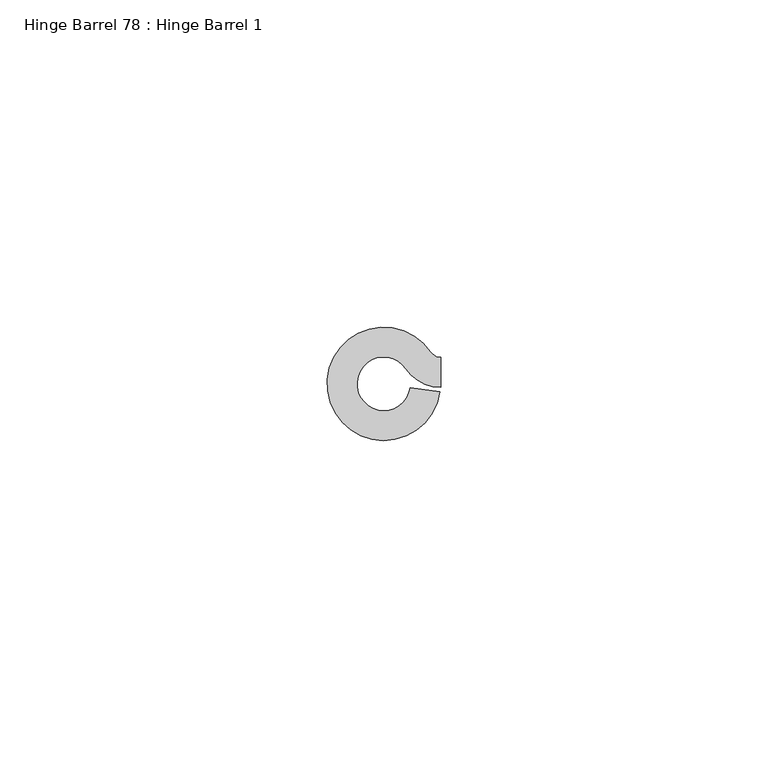
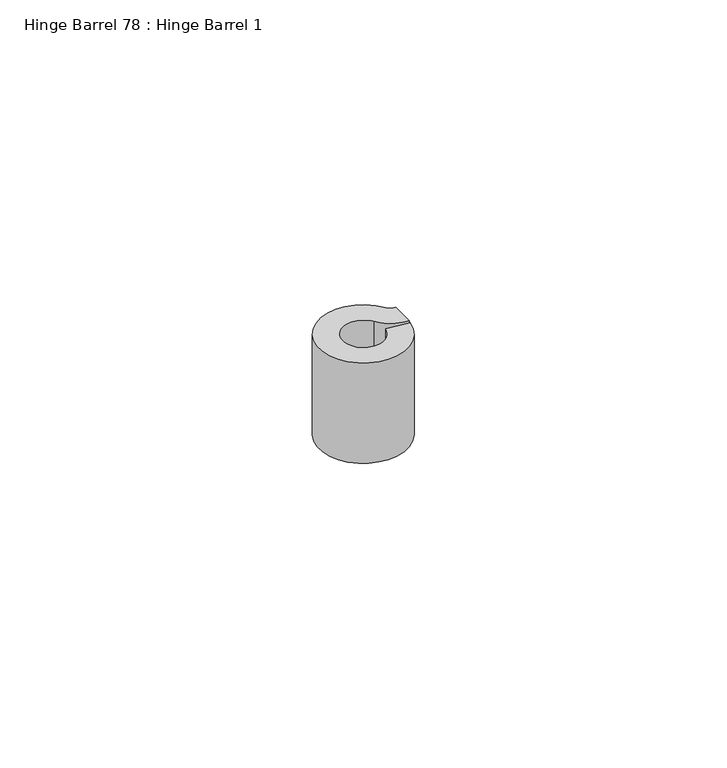
"""IFC4 building model written with IfcOpenShell, lengths in millimetres: proxy geometry, Hinge Barrel 78 : Hinge Barrel 1."""

from ifc_helpers import new_model, si_unit, point, frame, frame_2d, origin, place, context, project, spatial, polyline, circle_curve, trimmed, segment, composite_curve, outline, extrude, source, transform, mapped, element, save


def hinge_barrel_78_hinge_barrel_1_f6209b09(model_context):
    return source(origin(), model_context, "Body", "SweptSolid", [
        extrude(outline(composite_curve([segment(trimmed(circle_curve(frame_2d((587319.1320739, -531776.6049841)), 4.0894), [point((587322.5194669, -531774.3139665))], [point((587323.1821338, -531777.1708529))], True, "CARTESIAN"), True, "CONTINUOUS"), segment(polyline([(587323.1821338, -531777.1708529), (587327.7022899, -531777.8024028)]), True, "CONTINUOUS"), segment(trimmed(circle_curve(frame_2d((587319.1320739, -531776.6049841)), 8.6534625), [point((587327.7022899, -531777.8024028))], [point((587326.3000393, -531771.7570273))], False, "CARTESIAN"), True, "CONTINUOUS"), segment(trimmed(circle_curve(frame_2d((587327.8245257, -531770.7259615)), 1.8404226), [point((587326.3000393, -531771.7570273))], [point((587327.8245257, -531772.5663841))], True, "CARTESIAN"), True, "CONTINUOUS"), segment(polyline([(587327.8245257, -531772.5663841), (587327.8245257, -531777.1304466)]), True, "CONTINUOUS"), segment(trimmed(circle_curve(frame_2d((587327.8245257, -531770.7259615)), 6.4044851), [point((587327.8245257, -531777.1304466))], [point((587322.5194669, -531774.3139665))], False, "CARTESIAN"), True, "CONTINUOUS")], self_intersect=False)), frame((0.0, 0.0, 438.15), z_axis=(0.0, 0.0, 1.0), x_axis=(1.0, 0.0, 0.0)), (0.0, 0.0, 1.0), 20.8359375),
    ])


if __name__ == "__main__":
    model = new_model("IFC4")
    model_context = context("Model", 3, world=origin())
    ifc_project = project(units=[si_unit("LENGTHUNIT", "METRE", prefix="MILLI")], contexts=[model_context])
    site = spatial("IfcSite", under=ifc_project)
    building = spatial("IfcBuilding", under=site)
    placement = place(None, origin())
    hinge_barrel_78_hinge_barrel_1_shape = hinge_barrel_78_hinge_barrel_1_f6209b09(model_context)
    element("IfcBuildingElementProxy", 1, Name="Hinge Barrel 78 : Hinge Barrel 1", ObjectType="Hinge Barrel 78 : Hinge Barrel 1", at=placement, inside=building, context=model_context, shape_type="MappedRepresentation", body=[
        mapped(hinge_barrel_78_hinge_barrel_1_shape, transform((0.0, 0.0, 0.0), x_axis=(1.0, 0.0, 0.0), y_axis=(0.0, 1.0, 0.0), z_axis=(0.0, 0.0, 1.0))),
    ])
    save(model, "model.ifc")

# Revit data of these elements
# Element 1 (IfcBuildingElementProxy, "Hinge Barrel 78 : Hinge Barrel 1")
#   Materials on its faces: "6\"X6\" WELD-ON STL BUTT HINGE"
# Materials
#   "6\"X6\" WELD-ON STL BUTT HINGE": class "Metal", colour RGB 189 187 185, transparency 0, Description = "Carbon steel", Cost = 0
